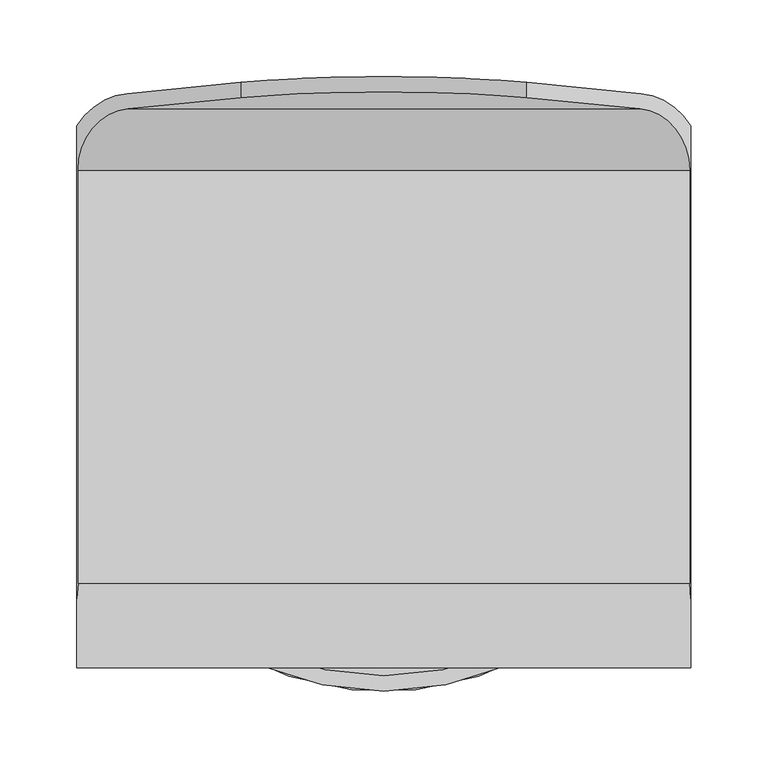
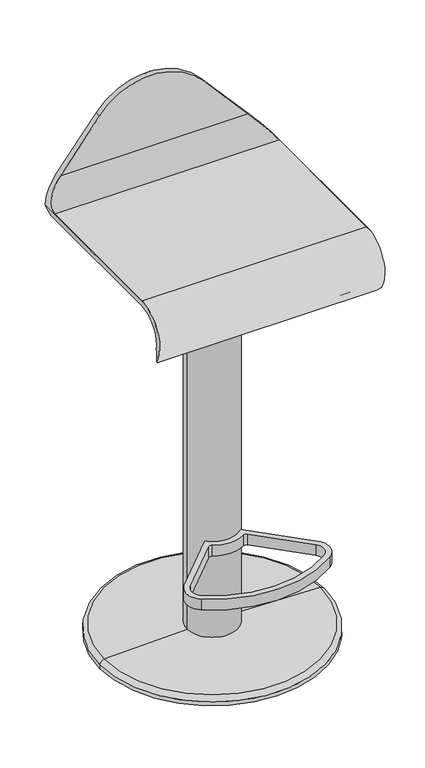
"""IFC4 building model written with IfcOpenShell, lengths in millimetres: furniture geometry, Allermuir_Surf_Stool_9179 : Allermuir_Surf_Stool_9179."""

from ifc_helpers import new_model, si_unit, point, frame, frame_2d, origin, place, context, project, spatial, polyline, circle_curve, ellipse_curve, trimmed, segment, composite_curve, outline, extrude, source, transform, mapped, element, save
from ifc_brep_helpers import plane_surface, cylinder_surface, revolved_surface, advanced_brep


def furniture_eb32228c(model_context):
    return source(origin(), model_context, "Body", "SolidModel", [
        extrude(outline(composite_curve([segment(trimmed(circle_curve(frame_2d((231.753449, 164.0039103)), 3.0), [point((229.7688585, 166.2536659))], [point((233.8747694, 166.1252306))], False, "CARTESIAN"), True, "CONTINUOUS"), segment(polyline([(233.8747694, 166.1252306), (318.3215957, 81.6784043)]), True, "CONTINUOUS"), segment(trimmed(circle_curve(frame_2d((297.1083922, 60.4652009)), 30.0), [point((318.3215957, 81.6784043))], [point((314.2451673, 35.8414128))], False, "CARTESIAN"), True, "CONTINUOUS"), segment(trimmed(circle_curve(frame_2d((200.0, 200.0)), 200.0), [point((314.2451673, 35.8414128))], [point((85.7548327, 35.8414128))], False, "CARTESIAN"), True, "CONTINUOUS"), segment(trimmed(circle_curve(frame_2d((102.8916078, 60.4652009)), 30.0), [point((85.7548327, 35.8414128))], [point((81.6784043, 81.6784043))], False, "CARTESIAN"), True, "CONTINUOUS"), segment(polyline([(81.6784043, 81.6784043), (166.1252306, 166.1252306)]), True, "CONTINUOUS"), segment(trimmed(circle_curve(frame_2d((168.246551, 164.0039103)), 3.0), [point((166.1252306, 166.1252306))], [point((170.2311415, 166.2536659))], False, "CARTESIAN"), True, "CONTINUOUS"), segment(trimmed(circle_curve(frame_2d((200.0, 200.0)), 45.0), [point((170.2311415, 166.2536659))], [point((229.7688585, 166.2536659))], True, "CARTESIAN"), True, "CONTINUOUS")], self_intersect=False), holes=[composite_curve([segment(polyline([(165.991876, 151.8497404), (88.7494721, 74.6073365)]), True, "CONTINUOUS"), segment(trimmed(circle_curve(frame_2d((102.8916078, 60.4652009)), 20.0), [point((88.7494721, 74.6073365))], [point((91.467091, 44.0493422))], True, "CARTESIAN"), True, "CONTINUOUS"), segment(trimmed(circle_curve(frame_2d((200.0, 200.0)), 190.0), [point((91.467091, 44.0493422))], [point((308.532909, 44.0493422))], True, "CARTESIAN"), True, "CONTINUOUS"), segment(trimmed(circle_curve(frame_2d((297.1083922, 60.4652009)), 20.0), [point((308.532909, 44.0493422))], [point((311.2505279, 74.6073365))], True, "CARTESIAN"), True, "CONTINUOUS"), segment(polyline([(311.2505279, 74.6073365), (234.008124, 151.8497404)]), True, "CONTINUOUS"), segment(trimmed(circle_curve(frame_2d((230.4725901, 148.3142065)), 5.0), [point((234.008124, 151.8497404))], [point((227.9332076, 152.6213559))], True, "CARTESIAN"), True, "CONTINUOUS"), segment(trimmed(circle_curve(frame_2d((200.0, 200.0)), 55.0), [point((227.9332076, 152.6213559))], [point((172.0667924, 152.6213559))], False, "CARTESIAN"), True, "CONTINUOUS"), segment(trimmed(circle_curve(frame_2d((169.5274099, 148.3142065)), 5.0), [point((172.0667924, 152.6213559))], [point((165.991876, 151.8497404))], True, "CARTESIAN"), True, "CONTINUOUS")], self_intersect=False)]), frame((0.0, 0.0, 180.0), z_axis=(0.0, 0.0, 1.0), x_axis=(1.0, 0.0, 0.0)), (0.0, 0.0, 1.0), 20.0),
        advanced_brep(
        [(245.0, 200.0, 20.0), (155.0, 200.0, 20.0), (155.0, 200.0, 0.0), (245.0, 200.0, 0.0), (392.041203, 200.0, 15.2567354), (7.958797, 200.0, 15.2567354), (400.0, 200.0, 0.0), (0.0, 200.0, 0.0), (0.0, 200.0, 7.0370632), (400.0, 200.0, 7.0370632)],
        [
            (0, 1, circle_curve(frame((200.0, 200.0, 20.0), z_axis=(0.0, 0.0, 1.0), x_axis=(-1.0, 0.0, 0.0)), 45.0)),
            (1, 2),
            (2, 3, circle_curve(frame((200.0, 200.0, 0.0), z_axis=(0.0, 0.0, -1.0), x_axis=(-1.0, 0.0, 0.0)), 45.0)),
            (3, 0),
            (1, 0, circle_curve(frame((200.0, 200.0, 20.0), z_axis=(0.0, 0.0, 1.0), x_axis=(-1.0, 0.0, 0.0)), 45.0)),
            (3, 2, circle_curve(frame((200.0, 200.0, 0.0), z_axis=(0.0, 0.0, -1.0), x_axis=(-1.0, 0.0, 0.0)), 45.0)),
            (4, 5, circle_curve(frame((200.0, 200.0, 15.2567354), z_axis=(0.0, 0.0, 1.0), x_axis=(-1.0, 0.0, 0.0)), 192.041203)),
            (5, 1),
            (0, 4),
            (5, 4, circle_curve(frame((200.0, 200.0, 15.2567354), z_axis=(0.0, 0.0, 1.0), x_axis=(-1.0, 0.0, 0.0)), 192.041203)),
            (6, 7, circle_curve(frame((200.0, 200.0, 0.0), z_axis=(0.0, 0.0, 1.0), x_axis=(-1.0, 0.0, 0.0)), 200.0)),
            (7, 8),
            (8, 9, circle_curve(frame((200.0, 200.0, 7.0370632), z_axis=(0.0, 0.0, -1.0), x_axis=(-1.0, 0.0, 0.0)), 200.0)),
            (9, 6),
            (7, 6, circle_curve(frame((200.0, 200.0, 0.0), z_axis=(0.0, 0.0, 1.0), x_axis=(-1.0, 0.0, 0.0)), 200.0)),
            (9, 8, circle_curve(frame((200.0, 200.0, 7.0370632), z_axis=(0.0, 0.0, -1.0), x_axis=(-1.0, 0.0, 0.0)), 200.0)),
            (2, 7),
            (6, 3),
            (8, 5, circle_curve(frame((8.2239477, 200.0, 7.0370632), z_axis=(0.0, 1.0, 0.0), x_axis=(1.0, 0.0, 0.0)), 8.2239477)),
            (4, 9, circle_curve(frame((391.7760523, 200.0, 7.0370632), z_axis=(0.0, 1.0, 0.0), x_axis=(-1.0, 0.0, 0.0)), 8.2239477)),
        ],
        [
            revolved_surface(polyline([(155.0, 200.0, 0.0), (155.0, 200.0, 20.0)]), (200.0, 200.0, 2438.4), (0.0, 0.0, -1.0)),
            revolved_surface(polyline([(155.0, 200.0, 20.0), (7.958797, 200.0, 15.2567354)]), (200.0, 200.0, 2438.4), (0.0, 0.0, -1.0)),
            cylinder_surface(frame((200.0, 200.0, 2438.4), z_axis=(0.0, 0.0, -1.0), x_axis=(-1.0, 0.0, 0.0)), 200.0),
            plane_surface(frame((200.0, 200.0, 0.0), z_axis=(0.0, 0.0, -1.0), x_axis=(-1.0, 0.0, 0.0))),
            revolved_surface(trimmed(ellipse_curve(frame((8.2239477, 200.0, 7.0370632), z_axis=(0.0, -1.0, 0.0), x_axis=(1.0, 0.0, 0.0)), 8.2239477, 8.2239477), [point((7.958797, 200.0, 15.2567354))], [point((0.0, 200.0, 7.0370632))], True, "CARTESIAN"), (200.0, 200.0, 2438.4), (0.0, 0.0, -1.0)),
        ],
        [
            (0, [[1, 2, 3, 4]]),
            (0, [[5, -4, 6, -2]]),
            (1, [[7, 8, -1, 9]]),
            (1, [[10, -9, -5, -8]]),
            (2, [[11, 12, 13, 14]]),
            (2, [[15, -14, 16, -12]]),
            (3, [[-3, 17, -11, 18]]),
            (3, [[-6, -18, -15, -17]]),
            (4, [[-13, 19, -7, 20]]),
            (4, [[-16, -20, -10, -19]]),
        ],
    ),
        advanced_brep(
        [(155.0, 200.0, 0.0), (245.0, 200.0, 0.0), (245.0, 200.0, 579.3900193), (155.0, 200.0, 579.3900193)],
        [
            (0, 1, circle_curve(frame((200.0, 200.0, 0.0), z_axis=(0.0, 0.0, -1.0), x_axis=(1.0, 0.0, 0.0)), 45.0)),
            (1, 0, circle_curve(frame((200.0, 200.0, 0.0), z_axis=(0.0, 0.0, -1.0), x_axis=(1.0, 0.0, 0.0)), 45.0)),
            (1, 2),
            (2, 3, ellipse_curve(frame((200.0, 200.0, 579.3900193), z_axis=(0.0, -0.5399439781834036, -0.8417009566487852), x_axis=(0.0, -0.8417009566487852, 0.5399439781834037)), 53.4631684, 45.0)),
            (3, 0),
            (3, 2, ellipse_curve(frame((200.0, 200.0, 579.3900193), z_axis=(0.0, -0.5399439781834036, -0.8417009566487852), x_axis=(0.0, -0.8417009566487852, 0.5399439781834037)), 53.4631684, 45.0)),
        ],
        [
            plane_surface(frame((245.0, 200.0, 0.0), z_axis=(0.0, 0.0, -1.0), x_axis=(0.0, -1.0, 0.0))),
            cylinder_surface(frame((200.0, 200.0, 0.0), z_axis=(0.0, 0.0, 1.0), x_axis=(1.0, 0.0, 0.0)), 45.0),
            plane_surface(frame((319.4506408, 140.0142682, 617.8703542), z_axis=(0.0, 0.5399439781834036, 0.8417009566487852), x_axis=(-1.0, 0.0, 0.0))),
        ],
        [
            (0, [[1, 2]]),
            (1, [[-2, 3, 4, 5]]),
            (1, [[-1, -5, 6, -3]]),
            (2, [[-4, -6]]),
        ],
    ),
        advanced_brep(
        [(400.0, 70.0919848, 760.0), (400.0, 339.3103685, 760.0), (400.0, 368.030606, 769.0714286), (400.0, 60.0281579, 769.0714286), (400.0, 25.0919848, 683.3772234), (400.0, 25.0919848, 705.2464075), (400.0, 26.1617284, 705.2464075), (0.0, 339.3103685, 760.0), (0.0, 70.0919848, 760.0), (0.0, 26.1617284, 705.2464075), (0.0, 25.0919848, 705.2464075), (0.0, 25.0919848, 683.3772234), (0.0, 60.0281579, 769.0714286), (0.0, 368.030606, 769.0714286), (367.2640038, 389.1201034, 805.6422129), (32.7359962, 389.1201034, 805.6422129), (106.8635277, 396.3651308, 888.4532553), (195.445222, 400.0, 930.0), (204.554778, 400.0, 930.0), (293.1364723, 396.3651308, 888.4532553), (33.5161627, 379.1581564, 806.5137703), (366.4838373, 379.1581564, 806.5137703), (293.1364723, 386.3269325, 888.4532553), (106.8635277, 386.3269325, 888.4532553), (0.831202, 339.3103685, 770.0), (399.168798, 339.3103685, 770.0), (0.831202, 70.0919848, 770.0), (399.168798, 70.0919848, 770.0), (11.5316988, 40.395066, 668.7064474), (388.4683012, 40.395066, 668.7064474), (156.0750469, 232.2105677, 545.6584406), (243.9249531, 232.2105677, 545.6584406), (245.0, 200.0, 566.3212448), (155.0, 200.0, 566.3212448), (15.6004685, 45.7945058, 677.123457), (384.3995315, 45.7945058, 677.123457), (243.9249531, 232.2105677, 557.5391447), (156.0750469, 232.2105677, 557.5391447), (155.0, 200.0, 578.2019489), (245.0, 200.0, 578.2019489), (399.1938904, 26.1617284, 705.2464075), (0.8061096, 26.1617284, 705.2464075)],
        [
            (0, 1),
            (1, 2, circle_curve(frame((400.0, 339.3103685, 810.0), z_axis=(1.0, 0.0, 0.0), x_axis=(0.0, -1.0, 0.0)), 50.0)),
            (2, 3),
            (3, 4, circle_curve(frame((400.0, 70.0919848, 715.0), z_axis=(1.0, 0.0, 0.0), x_axis=(0.0, -1.0, 0.0)), 55.0)),
            (4, 5),
            (5, 6),
            (6, 0, circle_curve(frame((400.0, 70.0919848, 715.0), z_axis=(-1.0, 0.0, 0.0), x_axis=(0.0, -1.0, 0.0)), 45.0)),
            (7, 8),
            (8, 9, circle_curve(frame((0.0, 70.0919848, 715.0), z_axis=(1.0, 0.0, 0.0), x_axis=(0.0, -1.0, 0.0)), 45.0)),
            (9, 10),
            (10, 11),
            (11, 12, circle_curve(frame((0.0, 70.0919848, 715.0), z_axis=(-1.0, 0.0, 0.0), x_axis=(0.0, -1.0, 0.0)), 55.0)),
            (12, 13),
            (13, 7, circle_curve(frame((0.0, 339.3103685, 810.0), z_axis=(-1.0, 0.0, 0.0), x_axis=(0.0, -1.0, 0.0)), 50.0)),
            (14, 15),
            (15, 16),
            (16, 17, ellipse_curve(frame((200.0, 389.0711796, 805.0830116), z_axis=(0.0, 0.9961946980917454, -0.08715574274765918), x_axis=(0.0, 0.08715574274765936, 0.9961946980917454)), 125.4774797, 125.0)),
            (17, 18),
            (18, 19, ellipse_curve(frame((200.0, 389.0711796, 805.0830116), z_axis=(0.0, 0.9961946980917454, -0.08715574274765918), x_axis=(0.0, 0.08715574274765936, 0.9961946980917454)), 125.4774797, 125.0)),
            (19, 14),
            (17, 18, ellipse_curve(frame((200.0, 1827.8077112, 805.0830116), z_axis=(0.0, 0.0871557427476659, 0.9961946980917449), x_axis=(0.0, 0.9961946980917449, -0.0871557427476659)), 1434.2141557, 125.0)),
            (20, 21),
            (21, 22),
            (22, 23, ellipse_curve(frame((200.0, 379.0329813, 805.0830116), z_axis=(0.0, -0.9961946980917454, 0.08715574274765944), x_axis=(0.0, 0.0871557427476591, 0.9961946980917454)), 125.4774797, 125.0)),
            (23, 20),
            (20, 24, ellipse_curve(frame((36.6368286, 339.3103685, 810.0), z_axis=(-0.745091778044962, 0.0, 0.6669619496566481), x_axis=(-0.666961949656648, 0.0, -0.745091778044962)), 53.6846616, 40.0)),
            (24, 25),
            (25, 21, ellipse_curve(frame((363.3631714, 339.3103685, 810.0), z_axis=(0.7450917780449817, 0.0, 0.6669619496566261), x_axis=(-0.6669619496566259, 0.0, 0.7450917780449818)), 53.6846616, 40.0)),
            (24, 26),
            (26, 27),
            (27, 25),
            (0, 8),
            (7, 1),
            (13, 15, ellipse_curve(frame((36.6368286, 339.3103685, 810.0), z_axis=(0.745091778044962, 0.0, -0.6669619496566481), x_axis=(0.666961949656648, 0.0, 0.745091778044962)), 67.1058271, 50.0)),
            (14, 2, ellipse_curve(frame((363.3631714, 339.3103685, 810.0), z_axis=(-0.7450917780449817, 0.0, -0.6669619496566261), x_axis=(0.6669619496566259, 0.0, -0.7450917780449818)), 67.1058271, 50.0)),
            (19, 22),
            (27, 3, ellipse_curve(frame((448.4015345, 70.0919848, 715.0), z_axis=(0.7450917780449817, 0.0, 0.6669619496566261), x_axis=(0.6669619496566259, 0.0, -0.7450917780449818)), 73.8164098, 55.0)),
            (23, 16),
            (12, 26, ellipse_curve(frame((-48.4015345, 70.0919848, 715.0), z_axis=(-0.745091778044962, 0.0, 0.6669619496566481), x_axis=(0.666961949656648, 0.0, 0.745091778044962)), 73.8164098, 55.0)),
            (11, 28, ellipse_curve(frame((33.9099323, 70.0919848, 715.0), z_axis=(0.798635510047292, -0.6018150231520493, 0.0), x_axis=(0.6018150231520494, 0.7986355100472919, 0.0)), 68.8674612, 55.0)),
            (28, 29),
            (29, 4, ellipse_curve(frame((366.0900677, 70.0919848, 715.0), z_axis=(-0.798635510047292, -0.6018150231520495, 0.0), x_axis=(0.6018150231520493, -0.7986355100472922, 0.0)), 68.8674612, 55.0)),
            (28, 30),
            (30, 31, ellipse_curve(frame((200.0, 199.1107414, 566.8916966), z_axis=(0.0, -0.5399439781834032, -0.8417009566487854), x_axis=(0.0, 0.8417009566487854, -0.5399439781834033)), 65.3438725, 55.0)),
            (31, 29),
            (32, 33, ellipse_curve(frame((200.0, 200.0, 566.3212448), z_axis=(0.0, 0.5399439781834032, 0.8417009566487854), x_axis=(0.0, -0.8417009566487854, 0.5399439781834033)), 53.4631684, 45.0)),
            (33, 32, ellipse_curve(frame((200.0, 200.0, 566.3212448), z_axis=(0.0, 0.5399439781834032, 0.8417009566487854), x_axis=(0.0, -0.8417009566487854, 0.5399439781834033)), 53.4631684, 45.0)),
            (34, 35),
            (35, 36),
            (36, 37, ellipse_curve(frame((200.0, 199.1107414, 578.7724007), z_axis=(0.0, 0.5399439781834033, 0.8417009566487854), x_axis=(0.0, 0.8417009566487854, -0.5399439781834032)), 65.3438725, 55.0)),
            (37, 34),
            (38, 39, ellipse_curve(frame((200.0, 200.0, 578.2019489), z_axis=(0.0, -0.5399439781834033, -0.8417009566487854), x_axis=(0.0, -0.8417009566487854, 0.5399439781834032)), 53.4631684, 45.0)),
            (39, 38, ellipse_curve(frame((200.0, 200.0, 578.2019489), z_axis=(0.0, -0.5399439781834033, -0.8417009566487854), x_axis=(0.0, -0.8417009566487854, 0.5399439781834032)), 53.4631684, 45.0)),
            (6, 40),
            (40, 35, ellipse_curve(frame((366.0900677, 70.0919848, 715.0), z_axis=(0.798635510047292, 0.6018150231520495, 0.0), x_axis=(-0.6018150231520493, 0.7986355100472922, 0.0)), 56.3461046, 45.0)),
            (34, 41, ellipse_curve(frame((33.9099323, 70.0919848, 715.0), z_axis=(-0.798635510047292, 0.6018150231520493, 0.0), x_axis=(-0.6018150231520494, -0.7986355100472919, 0.0)), 56.3461046, 45.0)),
            (41, 9),
            (5, 40),
            (41, 10),
            (30, 37),
            (36, 31),
            (32, 39),
            (38, 33),
        ],
        [
            plane_surface(frame((400.0, 400.0, 930.0), z_axis=(1.0, 0.0, 0.0), x_axis=(0.0, 0.08715574274765918, 0.9961946980917454))),
            plane_surface(frame((0.0, 400.0, 930.0), z_axis=(-1.0, 0.0, 0.0), x_axis=(0.0, -0.08715574274765918, -0.9961946980917454))),
            plane_surface(frame((400.0, 389.1201034, 805.6422129), z_axis=(0.0, 0.9961946980917454, -0.08715574274765918), x_axis=(-1.0, 0.0, 0.0))),
            plane_surface(frame((400.0, 400.0, 930.0), z_axis=(0.0, 0.0871557427476659, 0.9961946980917449), x_axis=(-1.0, 0.0, 0.0))),
            plane_surface(frame((400.0, 390.038053, 930.8715574), z_axis=(0.0, -0.9961946980917454, 0.08715574274765944), x_axis=(-1.0, 0.0, 0.0))),
            revolved_surface(polyline([(0.831202, 299.3103685, 810.0), (399.168798, 299.3103685, 810.0)]), (0.0, 339.3103685, 810.0), (-1.0, 0.0, 0.0)),
            plane_surface(frame((400.0, 339.3103685, 770.0), z_axis=(0.0, 0.0, 1.0), x_axis=(-1.0, 0.0, 0.0))),
            plane_surface(frame((400.0, 70.0919848, 760.0), z_axis=(0.0, 0.0, -1.0), x_axis=(-1.0, 0.0, 0.0))),
            cylinder_surface(frame((0.0, 339.3103685, 810.0), z_axis=(1.0, 0.0, 0.0), x_axis=(0.0, -1.0, 0.0)), 50.0),
            plane_surface(frame((293.1364723, -206.7636844, 888.4532553), z_axis=(0.7450917780449817, 0.0, 0.6669619496566261), x_axis=(0.0, 1.0, 0.0))),
            plane_surface(frame((-8.1202046, -206.7636844, 760.0), z_axis=(-0.745091778044962, 0.0, 0.6669619496566481), x_axis=(0.0, 1.0, 0.0))),
            cylinder_surface(frame((200.0, 480.8963376, 805.0830116), z_axis=(0.0, 1.0, 0.0), x_axis=(-1.0, 0.0, 0.0)), 125.0),
            cylinder_surface(frame((0.0, 70.0919848, 715.0), z_axis=(1.0, 0.0, 0.0), x_axis=(0.0, -1.0, 0.0)), 55.0),
            plane_surface(frame((400.0, 40.395066, 668.7064474), z_axis=(0.0, -0.5399439781834032, -0.8417009566487854), x_axis=(-1.0, 0.0, 0.0))),
            plane_surface(frame((400.0, 272.006426, 532.0104413), z_axis=(0.0, 0.5399439781834033, 0.8417009566487854), x_axis=(-1.0, 0.0, 0.0))),
            revolved_surface(polyline([(0.0, 25.091984800000006, 715.0), (400.0, 25.091984800000006, 715.0)]), (0.0, 70.0919848, 715.0), (-1.0, 0.0, 0.0)),
            plane_surface(frame((255.0, 199.1107414, 705.2464075), z_axis=(0.0, 0.0, -1.0), x_axis=(0.0, -1.0, 0.0))),
            cylinder_surface(frame((200.0, 199.1107414, 482.1686256), z_axis=(0.0, 0.0, -1.0), x_axis=(1.0, 0.0, 0.0)), 55.0),
            plane_surface(frame((243.9249531, 232.2105677, 705.2464075), z_axis=(0.798635510047292, 0.6018150231520495, 0.0), x_axis=(0.0, 0.0, -1.0))),
            plane_surface(frame((0.0, 25.0919848, 705.2464075), z_axis=(-0.798635510047292, 0.6018150231520493, 0.0), x_axis=(0.0, 0.0, -1.0))),
            revolved_surface(polyline([(245.0, 200.0, 607.0690647321853), (245.0, 200.0, 537.4541289678148)]), (200.0, 200.0, 482.1686256), (0.0, 0.0, 1.0)),
        ],
        [
            (0, [[1, 2, 3, 4, 5, 6, 7]]),
            (1, [[8, 9, 10, 11, 12, 13, 14]]),
            (2, [[15, 16, 17, 18, 19, 20]]),
            (3, [[-18, 21]]),
            (4, [[22, 23, 24, 25]]),
            (5, [[-22, 26, 27, 28]]),
            (6, [[-27, 29, 30, 31]]),
            (7, [[-1, 32, -8, 33]]),
            (8, [[-33, -14, 34, -15, 35, -2]]),
            (9, [[36, -23, -28, -31, 37, -3, -35, -20]]),
            (10, [[38, -16, -34, -13, 39, -29, -26, -25]]),
            (11, [[-36, -19, -21, -17, -38, -24]]),
            (12, [[-30, -39, -12, 40, 41, 42, -4, -37]]),
            (13, [[-41, 43, 44, 45], [46, 47]]),
            (14, [[48, 49, 50, 51], [52, 53]]),
            (15, [[-32, -7, 54, 55, -48, 56, 57, -9]]),
            (16, [[58, -54, -6]]),
            (16, [[59, -10, -57]]),
            (17, [[60, -50, 61, -44]]),
            (18, [[-58, -5, -42, -45, -61, -49, -55]]),
            (19, [[-59, -56, -51, -60, -43, -40, -11]]),
            (20, [[62, -52, 63, -46]]),
            (20, [[-62, -47, -63, -53]]),
        ],
    ),
    ])


if __name__ == "__main__":
    model = new_model("IFC4")
    model_context = context("Model", 3, world=origin())
    ifc_project = project(units=[si_unit("LENGTHUNIT", "METRE", prefix="MILLI")], contexts=[model_context])
    site = spatial("IfcSite", under=ifc_project)
    building = spatial("IfcBuilding", under=site)
    placement = place(None, origin())
    furniture_shape = furniture_eb32228c(model_context)
    element("IfcFurniture", 1, ObjectType="Allermuir_Surf_Stool_9179 : Allermuir_Surf_Stool_9179", at=placement, inside=building, context=model_context, shape_type="MappedRepresentation", body=[
        mapped(furniture_shape, transform((0.0, 0.0, 0.0), x_axis=(1.0, 0.0, 0.0), y_axis=(0.0, 1.0, 0.0), z_axis=(0.0, 0.0, 1.0))),
    ])
    save(model, "model.ifc")

# Revit data of these elements
# Type "Allermuir_Surf_Stool_9179 : Allermuir_Surf_Stool_9179"
#   Support = chrome
#   Seat = orange paint
#   Base = chrome
#   Default Elevation = 0
# Element 1 (IfcFurniture, "Allermuir_Surf_Stool_9179 : Allermuir_Surf_Stool_9179")
#   Materials on its faces: "chrome", "orange paint"
# Materials
#   "chrome": class "Metal", colour RGB 244 244 244, transparency 0
#   "orange paint": class "Paint", colour RGB 248 199 146, transparency 0
